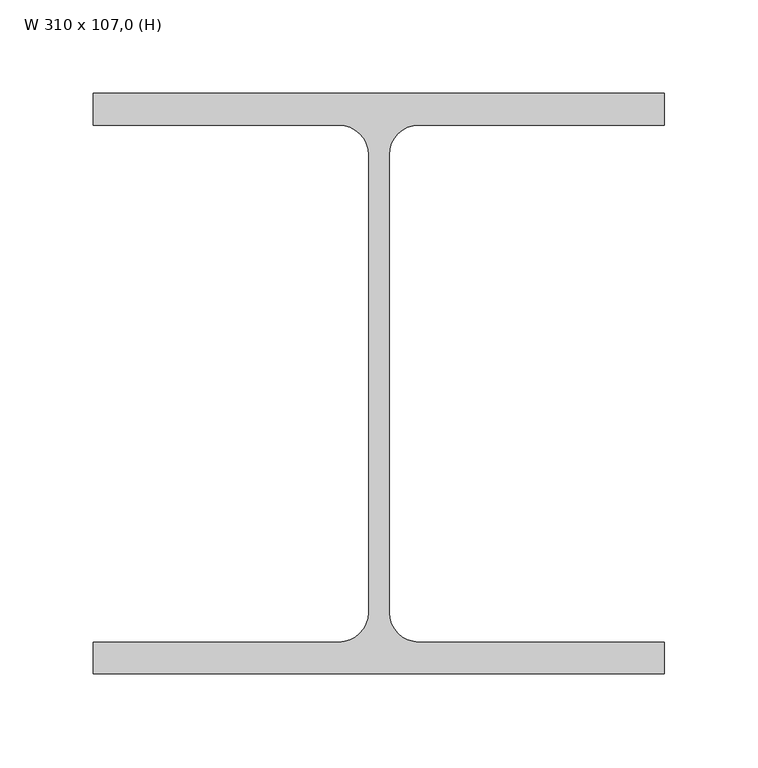
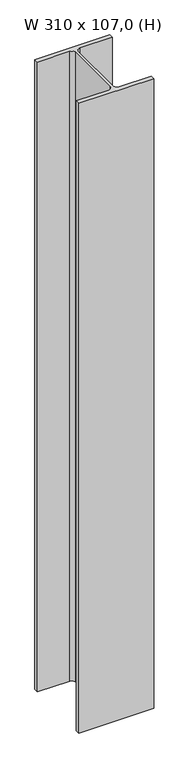
"""IFC4 building model written with IfcOpenShell, lengths in millimetres: column geometry, Pilar de Aço - H : W 310 x 107,0 (H)."""

from ifc_helpers import new_model, si_unit, point, frame_2d, origin, origin_with_axes, place, context, project, spatial, polyline, circle_curve, trimmed, segment, composite_curve, outline, extrude, source, transform, mapped, element, save


def w_310_x_107_0_h_c68161b5(model_context):
    return source(origin(), model_context, "Body", "SweptSolid", [
        extrude(outline(composite_curve([segment(polyline([(153.0, 155.5), (153.0, 138.5), (21.45, 138.5)]), True, "CONTINUOUS"), segment(trimmed(circle_curve(frame_2d((21.45, 122.5)), 16.0), [point((21.45, 138.5))], [point((5.45, 122.5))], True, "CARTESIAN"), True, "CONTINUOUS"), segment(polyline([(5.45, 122.5), (5.45, -122.5)]), True, "CONTINUOUS"), segment(trimmed(circle_curve(frame_2d((21.45, -122.5)), 16.0), [point((5.45, -122.5))], [point((21.45, -138.5))], True, "CARTESIAN"), True, "CONTINUOUS"), segment(polyline([(21.45, -138.5), (153.0, -138.5), (153.0, -155.5), (-153.0, -155.5), (-153.0, -138.5), (-21.45, -138.5)]), True, "CONTINUOUS"), segment(trimmed(circle_curve(frame_2d((-21.45, -122.5)), 16.0), [point((-21.45, -138.5))], [point((-5.45, -122.5))], True, "CARTESIAN"), True, "CONTINUOUS"), segment(polyline([(-5.45, -122.5), (-5.45, 122.5)]), True, "CONTINUOUS"), segment(trimmed(circle_curve(frame_2d((-21.45, 122.5)), 16.0), [point((-5.45, 122.5))], [point((-21.45, 138.5))], True, "CARTESIAN"), True, "CONTINUOUS"), segment(polyline([(-21.45, 138.5), (-153.0, 138.5), (-153.0, 155.5), (153.0, 155.5)]), True, "CONTINUOUS")], self_intersect=False)), origin_with_axes(), (0.0, 0.0, 1.0), 2720.0),
    ])


if __name__ == "__main__":
    model = new_model("IFC4")
    model_context = context("Model", 3, world=origin())
    ifc_project = project(units=[si_unit("LENGTHUNIT", "METRE", prefix="MILLI")], contexts=[model_context])
    site = spatial("IfcSite", under=ifc_project)
    building = spatial("IfcBuilding", under=site)
    placement = place(None, origin())
    w_310_x_107_0_h_shape = w_310_x_107_0_h_c68161b5(model_context)
    element("IfcColumn", 1, ObjectType="Pilar de Aço - H : W 310 x 107,0 (H)", at=placement, inside=building, context=model_context, shape_type="MappedRepresentation", body=[
        mapped(w_310_x_107_0_h_shape, transform((0.0, 0.0, 0.0), x_axis=(1.0, 0.0, 0.0), y_axis=(0.0, 1.0, 0.0), z_axis=(0.0, 0.0, 1.0))),
    ])
    save(model, "model.ifc")

# Revit data of these elements
# Type "Pilar de Aço - H : W 310 x 107,0 (H)"
#   SINAPI = ""
#   Área da seção = 136.4 m²
#   tw = 1.09 cm
#   tf = 1.70 cm
#   h = 27.70 cm
#   d' = 24.50 cm
#   d = 31.10 cm
#   bf = 30.60 cm
#   R = 1.60 cm
#   Massa Linear kg/m = 107
#   Aço = Metal - Aço 345MPa
#   Assembly Code = ""
# Materials
#   "Metal - Aço 345MPa": class "Metal", colour RGB 189 187 185, transparency 0, Cost = 0
